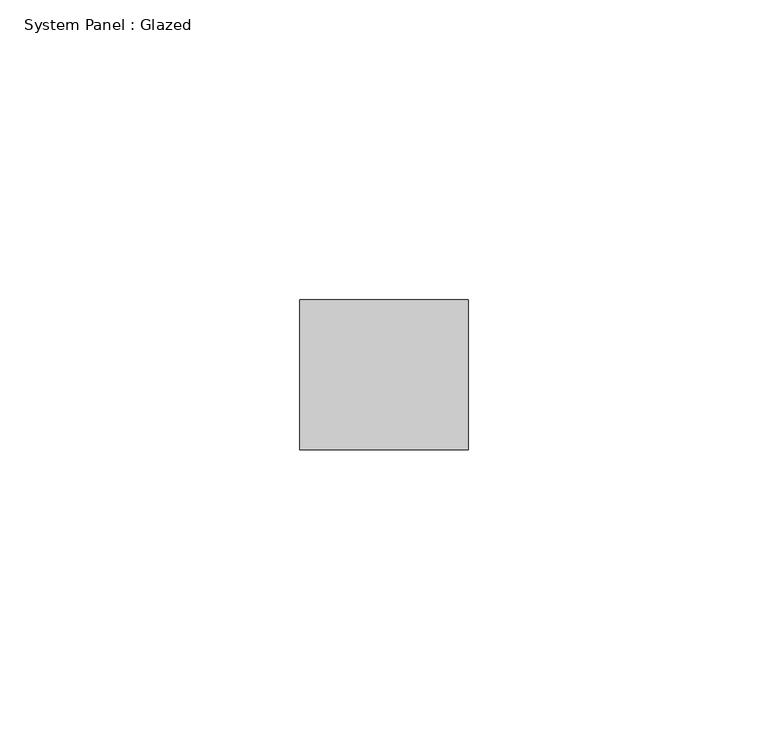
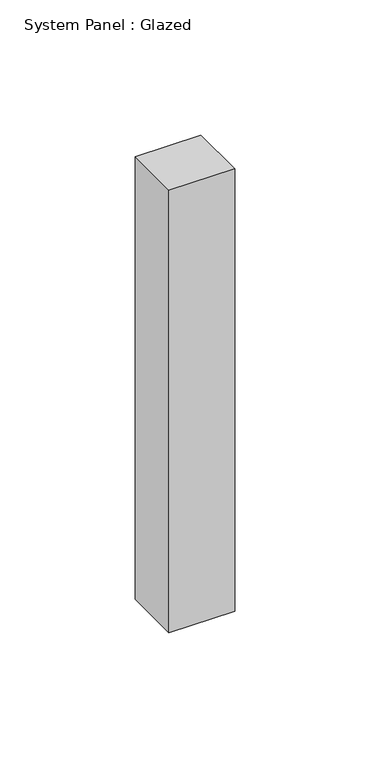
"""IFC4 building model written with IfcOpenShell, lengths in millimetres: plate geometry, System Panel : Glazed."""

from ifc_helpers import new_model, si_unit, origin, origin_with_axes, place, context, project, spatial, polyline, outline, extrude, source, transform, mapped, element, save


def system_panel_glazed_acae83c8(model_context):
    return source(origin(), model_context, "Body", "SweptSolid", [
        extrude(outline(polyline([(14.0474574, 24.5), (-14.0474574, 24.5), (-14.0474574, 49.5), (14.0474574, 49.5), (14.0474574, 24.5)])), origin_with_axes(), (0.0, 0.0, 1.0), 200.0),
    ])


if __name__ == "__main__":
    model = new_model("IFC4")
    model_context = context("Model", 3, world=origin())
    ifc_project = project(units=[si_unit("LENGTHUNIT", "METRE", prefix="MILLI")], contexts=[model_context])
    site = spatial("IfcSite", under=ifc_project)
    building = spatial("IfcBuilding", under=site)
    placement = place(None, origin())
    system_panel_glazed_shape = system_panel_glazed_acae83c8(model_context)
    element("IfcPlate", 1, ObjectType="System Panel : Glazed", at=placement, inside=building, context=model_context, shape_type="MappedRepresentation", body=[
        mapped(system_panel_glazed_shape, transform((0.0, 0.0, 0.0), x_axis=(1.0, 0.0, 0.0), y_axis=(0.0, 1.0, 0.0), z_axis=(0.0, 0.0, 1.0))),
    ])
    save(model, "model.ifc")

# Revit data of these elements
# Element 1 (IfcPlate, "System Panel : Glazed")
#   Materials on its faces: "Glass"
# Materials
#   "Glass": class "Glass", colour RGB 218 227 224, transparency 0.85, Description = "Soda Lime Glass", Cost = 0
